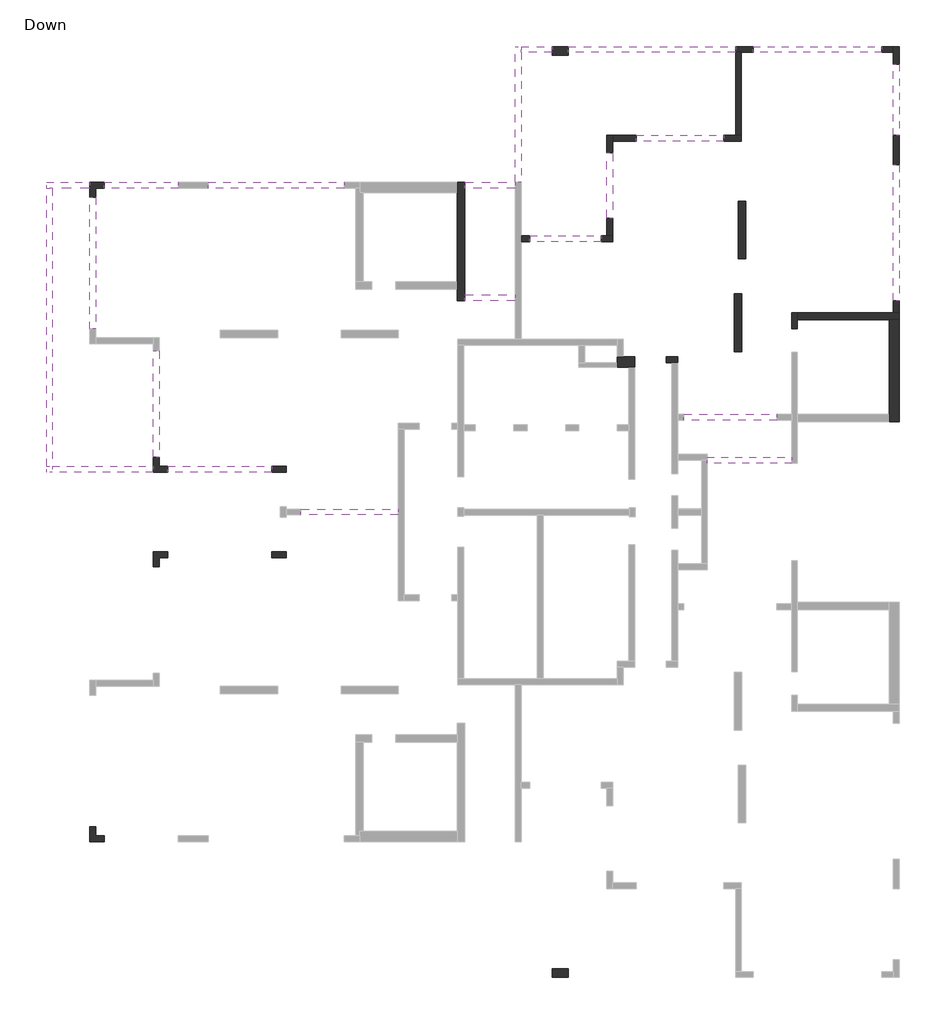
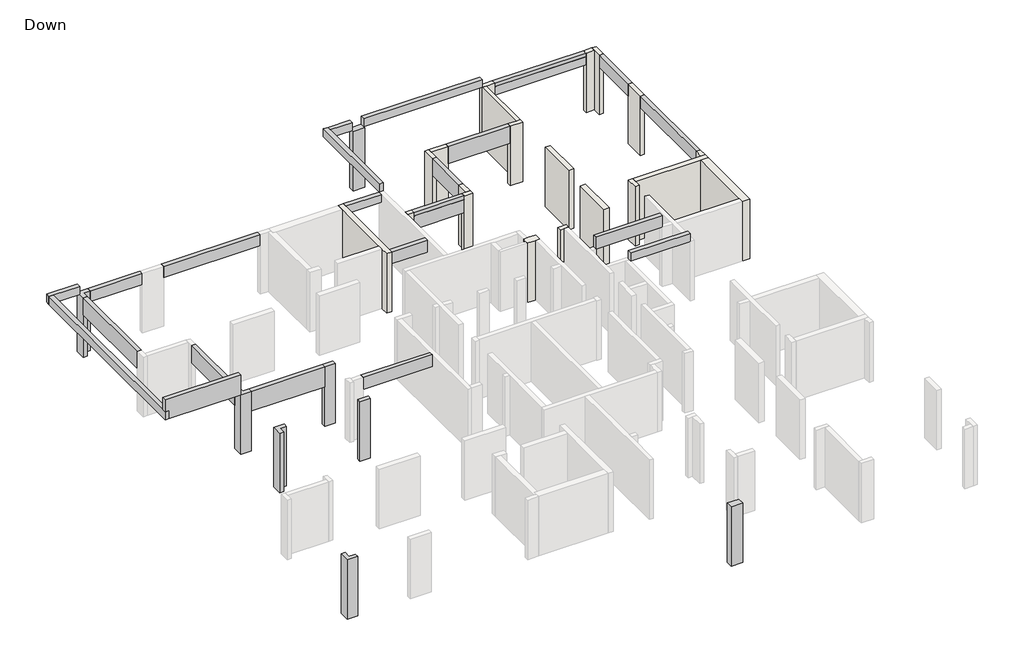
# One storey, part 3 of 3: 22 beams, 20 walls, 8 columns.
# Revit data of these elements (continued)
# Element 44 (IfcWall, "20") (continued)
#   Top Constraint = Typical Floor
#   Materials on its faces: "Concrete"
# Element 45 (IfcWall, "25")
#   Comments = ""
#   Mark = "W88"
#   SOFiSTiK_EdgeZones = "W88"
#   SOFiSTiK_AMG_Comments = ""
#   Top Offset = 0 cm
#   Base Offset = 0 cm
#   wall height = 300 cm
#   SOFiSTiK_AMG_Scheduled = yes
#   SOFiSTiK_AMG_Adjusted = yes
#   Phase Created = New Construction
#   Base Constraint = Down
#   Top Constraint = Typical Floor
#   Materials on its faces: "Concrete"
# Element 46 (IfcWall, "25")
#   Comments = ""
#   Mark = "W92"
#   SOFiSTiK_EdgeZones = "W92"
#   SOFiSTiK_AMG_Comments = ""
#   Top Offset = 0 cm
#   Base Offset = 0 cm
#   wall height = 300 cm
#   SOFiSTiK_AMG_Scheduled = yes
#   SOFiSTiK_AMG_Adjusted = yes
#   Phase Created = New Construction
#   Base Constraint = Down
#   Top Constraint = Typical Floor
#   Materials on its faces: "Concrete"
# Element 47 (IfcWall, "25")
#   Comments = ""
#   Mark = "W93"
#   SOFiSTiK_EdgeZones = "W93"
#   SOFiSTiK_AMG_Comments = ""
#   Top Offset = 0 cm
#   Base Offset = 0 cm
#   wall height = 300 cm
#   SOFiSTiK_AMG_Scheduled = yes
#   SOFiSTiK_AMG_Adjusted = yes
#   Phase Created = New Construction
#   Base Constraint = Down
#   Top Constraint = Typical Floor
#   Materials on its faces: "Concrete"
# Element 48 (IfcWall, "25")
#   Comments = ""
#   Mark = "W94"
#   SOFiSTiK_EdgeZones = "W94"
#   SOFiSTiK_AMG_Comments = ""
#   Top Offset = 0 cm
#   Base Offset = 0 cm
#   wall height = 300 cm
#   SOFiSTiK_AMG_Scheduled = yes
#   SOFiSTiK_AMG_Adjusted = yes
#   Phase Created = New Construction
#   Base Constraint = Down
#   Top Constraint = Typical Floor
#   Materials on its faces: "Concrete"
# Element 49 (IfcWall, "35")
#   Comments = ""
#   Mark = "W108"
#   SOFiSTiK_EdgeZones = "W108"
#   SOFiSTiK_AMG_Comments = ""
#   Top Offset = 0 cm
#   Base Offset = 0 cm
#   wall height = 300 cm
#   SOFiSTiK_AMG_Scheduled = yes
#   SOFiSTiK_AMG_Adjusted = yes
#   Phase Created = New Construction
#   Base Constraint = Down
#   Top Constraint = Typical Floor
#   Materials on its faces: "Concrete"
# Element 50 (IfcWall, "35")
#   Comments = ""
#   Mark = "W109"
#   SOFiSTiK_EdgeZones = "W109"
#   SOFiSTiK_AMG_Comments = ""
#   Top Offset = 0 cm
#   Base Offset = 0 cm
#   wall height = 300 cm
#   SOFiSTiK_AMG_Scheduled = yes
#   SOFiSTiK_AMG_Adjusted = yes
#   Phase Created = New Construction
#   Base Constraint = Down
#   Top Constraint = Typical Floor
#   Materials on its faces: "Concrete"
# Materials
#   "Concrete": class "Concrete", colour RGB 192 192 192, transparency 0, Keynote = "01000", Description = "Cast-in-place concrete", Cost = 0
#   "Concrete, Cast-in-Place gray": class "Concrete", colour RGB 192 192 192, transparency 0, Description = "Cast-in-place concrete", Cost = 0
